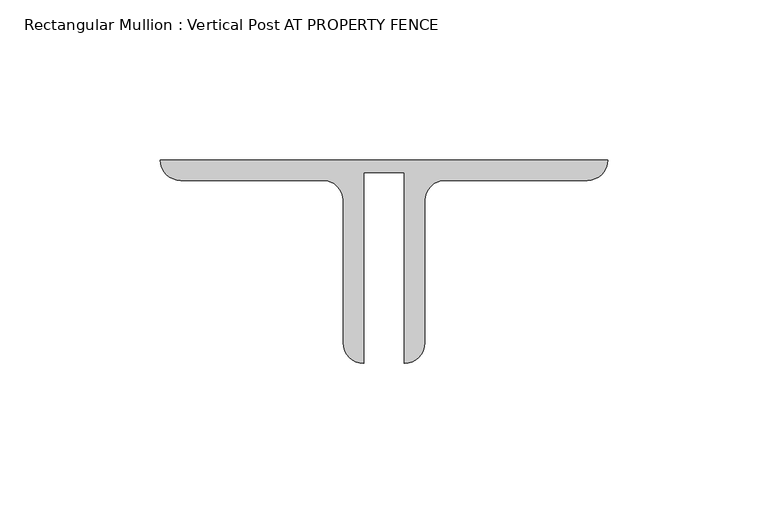
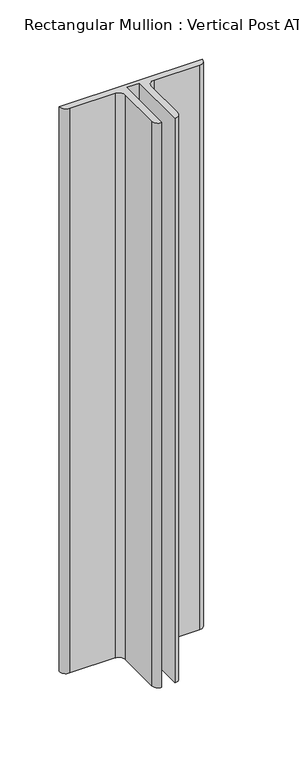
"""IFC4 building model written with IfcOpenShell, lengths in millimetres: member geometry, Rectangular Mullion : Vertical Post AT PROPERTY FENCE."""

from ifc_helpers import new_model, si_unit, point, frame, frame_2d, origin, place, context, project, spatial, polyline, circle_curve, trimmed, segment, composite_curve, outline, extrude, source, transform, mapped, element, save


def rectangular_mullion_vertical_post_at_property_fence_cb7719b9(model_context):
    return source(origin(), model_context, "Body", "SweptSolid", [
        extrude(outline(composite_curve([segment(polyline([(-63.5, -22.9145205), (-76.2, -22.9145205), (-76.2, -82.55)]), True, "CONTINUOUS"), segment(trimmed(circle_curve(frame_2d((-76.2, -76.2)), 6.35), [point((-76.2, -82.55))], [point((-82.55, -76.2))], False, "CARTESIAN"), True, "CONTINUOUS"), segment(polyline([(-82.55, -76.2), (-82.55, -31.75)]), True, "CONTINUOUS"), segment(trimmed(circle_curve(frame_2d((-88.9, -31.75)), 6.35), [point((-82.55, -31.75))], [point((-88.9, -25.4))], True, "CARTESIAN"), True, "CONTINUOUS"), segment(polyline([(-88.9, -25.4), (-133.35, -25.4)]), True, "CONTINUOUS"), segment(trimmed(circle_curve(frame_2d((-133.35, -19.05)), 6.35), [point((-133.35, -25.4))], [point((-139.7, -19.05))], False, "CARTESIAN"), True, "CONTINUOUS"), segment(polyline([(-139.7, -19.05), (0.0, -19.05)]), True, "CONTINUOUS"), segment(trimmed(circle_curve(frame_2d((-6.35, -19.05)), 6.35), [point((0.0, -19.05))], [point((-6.35, -25.4))], False, "CARTESIAN"), True, "CONTINUOUS"), segment(polyline([(-6.35, -25.4), (-50.8, -25.4)]), True, "CONTINUOUS"), segment(trimmed(circle_curve(frame_2d((-50.8, -31.75)), 6.35), [point((-50.8, -25.4))], [point((-57.15, -31.75))], True, "CARTESIAN"), True, "CONTINUOUS"), segment(polyline([(-57.15, -31.75), (-57.15, -76.2)]), True, "CONTINUOUS"), segment(trimmed(circle_curve(frame_2d((-63.5, -76.2)), 6.35), [point((-57.15, -76.2))], [point((-63.5, -82.55))], False, "CARTESIAN"), True, "CONTINUOUS"), segment(polyline([(-63.5, -82.55), (-63.5, -22.9145205)]), True, "CONTINUOUS")], self_intersect=False)), frame((0.0, 0.0, -581.9336948), z_axis=(0.0, 0.0, 1.0), x_axis=(1.0, 0.0, 0.0)), (0.0, 0.0, 1.0), 581.9336948),
    ])


if __name__ == "__main__":
    model = new_model("IFC4")
    model_context = context("Model", 3, world=origin())
    ifc_project = project(units=[si_unit("LENGTHUNIT", "METRE", prefix="MILLI")], contexts=[model_context])
    site = spatial("IfcSite", under=ifc_project)
    building = spatial("IfcBuilding", under=site)
    placement = place(None, origin())
    rectangular_mullion_vertical_post_at_property_fence_shape = rectangular_mullion_vertical_post_at_property_fence_cb7719b9(model_context)
    element("IfcMember", 1, ObjectType="Rectangular Mullion : Vertical Post AT PROPERTY FENCE", at=placement, inside=building, context=model_context, shape_type="MappedRepresentation", body=[
        mapped(rectangular_mullion_vertical_post_at_property_fence_shape, transform((0.0, 0.0, 0.0), x_axis=(1.0, 0.0, 0.0), y_axis=(0.0, 1.0, 0.0), z_axis=(0.0, 0.0, 1.0))),
    ])
    save(model, "model.ifc")

# Revit data of these elements
# Type "Rectangular Mullion : Vertical Post AT PROPERTY FENCE"
#   built-in parameter 1007351 = -0.0625 (stored number, unit not read)
#   built-in parameter 1007322 = 0.0126789 (stored number, unit not read)
#   built-in parameter 1007321 = 0.229167 (stored number, unit not read)
#   built-in parameter 1007320 = 0.229167 (stored number, unit not read)
# Element 1 (IfcMember, "Rectangular Mullion : Vertical Post AT PROPERTY FENCE")
#   Materials on its faces: "MAIN FENCE POST: (2) BACK/BACK GALVANIZED ANGLES (2) L2 1/2 X 2 1/2 X 1/4\") ANCHORED TO 8\"W X 42\" DEEP CONCRETE FOOTING(1)"
# Materials
#   "MAIN FENCE POST: (2) BACK/BACK GALVANIZED ANGLES (2) L2 1/2 X 2 1/2 X 1/4\") ANCHORED TO 8\"W X 42\" DEEP CONCRETE FOOTING(1)": class "Unassigned", colour RGB 211 211 211, transparency 0, Cost = 0
